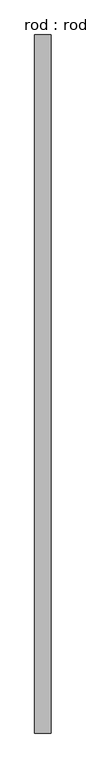
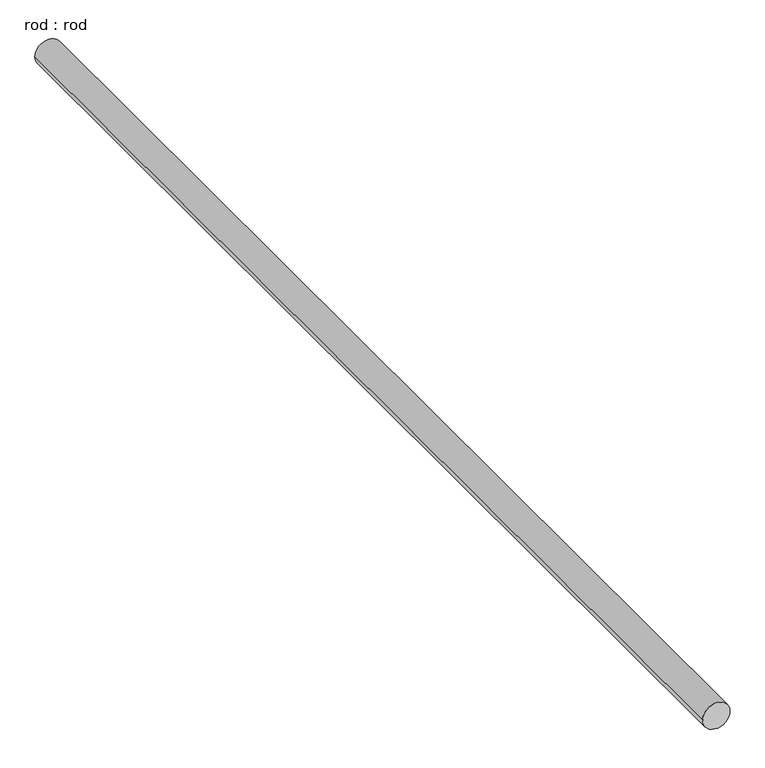
"""IFC4 building model written with IfcOpenShell, lengths in millimetres: proxy geometry, rod : rod."""

import ifcopenshell
import ifcopenshell.guid

model = None  # the IFC model being written
_history = None  # IfcOwnerHistory: only IFC2X3 demands one
_inside = {}  # id of a spatial element -> (the spatial element, [elements in it])
_under = {}  # id of a project, library or spatial element -> (it, [spatial elements below it])
_declared = {}  # id of a project -> (the project, [libraries it declares])
_typed = {}  # id of a type object -> (the type object, [elements of that type])
_made_of = {}  # id of a material, layer set ... -> (it, [elements and type objects made of it])


def new_model(schema):
    """Start an empty IFC model of exactly this schema.

    Asked for "IFC4X3", IfcOpenShell would pick the latest addendum, in which some entities
    have other attributes; the version numbers below select the first issue.
    IFC2X3 requires an IfcOwnerHistory on every rooted entity: one is made here for all.
    """
    global model, _history
    if schema == "IFC4X3":
        model = ifcopenshell.file(schema_version=(4, 3, 0, 0))
    else:
        model = ifcopenshell.file(schema=schema)
    _inside.clear()
    _under.clear()
    _declared.clear()
    _typed.clear()
    _made_of.clear()
    _history = None
    if model.schema == "IFC2X3":
        org = make("IfcOrganization", Name="unknown")
        user = make(
            "IfcPersonAndOrganization",
            ThePerson=make("IfcPerson", FamilyName="unknown"),
            TheOrganization=org,
        )
        app = make(
            "IfcApplication",
            ApplicationDeveloper=org,
            Version="unknown",
            ApplicationFullName="unknown",
            ApplicationIdentifier="unknown",
        )
        _history = make(
            "IfcOwnerHistory",
            OwningUser=user,
            OwningApplication=app,
            ChangeAction="ADDED",
            CreationDate=0,
        )
    return model


def make(cls, **values):
    """One entity of the class cls with the attributes given. An attribute that is None is left unset."""
    return model.create_entity(
        cls, **{name: value for name, value in values.items() if value is not None}
    )


def rooted(cls, **values):
    """An entity with a GlobalId (a new one), such as an element, a storey or a relation."""
    return make(cls, GlobalId=ifcopenshell.guid.new(), OwnerHistory=_history, **values)


def si_unit(unit_type, name, prefix=None):
    """IfcSIUnit, for example si_unit("LENGTHUNIT", "METRE", prefix="MILLI")."""
    return make("IfcSIUnit", UnitType=unit_type, Prefix=prefix, Name=name)


def assignment(units):
    """IfcUnitAssignment: the units of a project."""
    return None if units is None else make("IfcUnitAssignment", Units=units)


def point(xyz):
    """IfcCartesianPoint."""
    return None if xyz is None else make("IfcCartesianPoint", Coordinates=xyz)


def direction(xyz):
    """IfcDirection."""
    return None if xyz is None else make("IfcDirection", DirectionRatios=xyz)


def frame(location, z_axis=None, x_axis=None):
    """IfcAxis2Placement3D, a coordinate frame: its origin and axes. An axis left out is left unset."""
    return make(
        "IfcAxis2Placement3D",
        Location=point(location),
        Axis=direction(z_axis),
        RefDirection=direction(x_axis),
    )


def frame_2d(location, x_axis=None):
    """IfcAxis2Placement2D, a coordinate frame in the plane: its origin and x axis."""
    return make(
        "IfcAxis2Placement2D", Location=point(location), RefDirection=direction(x_axis)
    )


def origin():
    """The frame at (0, 0, 0) with its axes left unset."""
    return frame((0.0, 0.0, 0.0))


def place(relative_to, where):
    """IfcLocalPlacement: puts the frame where relative to a parent placement (None: the world)."""
    return make(
        "IfcLocalPlacement", PlacementRelTo=relative_to, RelativePlacement=where
    )


def context(
    kind, dimensions, precision=None, world=None, true_north=None, identifier=None
):
    """IfcGeometricRepresentationContext, for example the 3D "Model" context."""
    return make(
        "IfcGeometricRepresentationContext",
        ContextIdentifier=identifier,
        ContextType=kind,
        CoordinateSpaceDimension=dimensions,
        Precision=precision,
        WorldCoordinateSystem=world,
        TrueNorth=true_north,
    )


def project(units=None, contexts=None):
    """IfcProject with its units and contexts."""
    return rooted(
        "IfcProject",
        Name="project",
        RepresentationContexts=contexts,
        UnitsInContext=assignment(units),
    )


def spatial(cls, under=None, at=None, **own):
    """A site, building, storey or space (cls), placed at a placement, below another one or the project."""
    s = rooted(cls, ObjectPlacement=at, **own)
    if under is not None:
        _under.setdefault(under.id(), (under, []))[1].append(s)
    return s


def circle_curve(where, radius):
    """IfcCircle in the frame where."""
    return make("IfcCircle", Position=where, Radius=radius)


def trimmed(basis, trim1, trim2, sense, master):
    """IfcTrimmedCurve: the piece of a basis curve between two trims."""
    return make(
        "IfcTrimmedCurve",
        BasisCurve=basis,
        Trim1=trim1,
        Trim2=trim2,
        SenseAgreement=sense,
        MasterRepresentation=master,
    )


def segment(curve, same_sense, transition):
    """IfcCompositeCurveSegment."""
    return make(
        "IfcCompositeCurveSegment",
        Transition=transition,
        SameSense=same_sense,
        ParentCurve=curve,
    )


def composite_curve(segments, self_intersect=None):
    """IfcCompositeCurve: segments joined end to end."""
    return make("IfcCompositeCurve", Segments=segments, SelfIntersect=self_intersect)


def outline(outer, holes=None, kind="AREA"):
    """IfcArbitraryClosedProfileDef: a profile drawn as a closed curve; with holes, ...WithVoids."""
    if holes is None:
        return make("IfcArbitraryClosedProfileDef", ProfileType=kind, OuterCurve=outer)
    return make(
        "IfcArbitraryProfileDefWithVoids",
        ProfileType=kind,
        OuterCurve=outer,
        InnerCurves=holes,
    )


def extrude(swept, where, along, depth):
    """IfcExtrudedAreaSolid: the profile swept, set in the frame where, extruded along a direction by depth."""
    return make(
        "IfcExtrudedAreaSolid",
        SweptArea=swept,
        Position=where,
        ExtrudedDirection=direction(along),
        Depth=depth,
    )


def shape(context_of_items, identifier, shape_type, items):
    """IfcShapeRepresentation: the items that make up one representation, for example the "Body"."""
    return make(
        "IfcShapeRepresentation",
        ContextOfItems=context_of_items,
        RepresentationIdentifier=identifier,
        RepresentationType=shape_type,
        Items=items,
    )


def source(mapping_origin, context_of_items, identifier, shape_type, items):
    """IfcRepresentationMap: a shape defined once, which mapped items show again and again."""
    return make(
        "IfcRepresentationMap",
        MappingOrigin=mapping_origin,
        MappedRepresentation=shape(context_of_items, identifier, shape_type, items),
    )


def transform(
    local_origin,
    x_axis=None,
    y_axis=None,
    z_axis=None,
    scale=None,
    scale2=None,
    scale3=None,
    uniform=True,
):
    """IfcCartesianTransformationOperator3D, or its non-uniform kind. x_axis, y_axis, z_axis: its Axis1, 2, 3."""
    if uniform:
        return make(
            "IfcCartesianTransformationOperator3D",
            Axis1=direction(x_axis),
            Axis2=direction(y_axis),
            LocalOrigin=point(local_origin),
            Scale=scale,
            Axis3=direction(z_axis),
        )
    return make(
        "IfcCartesianTransformationOperator3DnonUniform",
        Axis1=direction(x_axis),
        Axis2=direction(y_axis),
        LocalOrigin=point(local_origin),
        Scale=scale,
        Axis3=direction(z_axis),
        Scale2=scale2,
        Scale3=scale3,
    )


def mapped(mapping_source, mapping_target):
    """IfcMappedItem: shows the shape of a source again, moved by a transform."""
    return make(
        "IfcMappedItem", MappingSource=mapping_source, MappingTarget=mapping_target
    )


def made_of(thing, what):
    """Note that an element or type object is made of a material, layer set ...; save() writes the relation."""
    if what is not None:
        _made_of.setdefault(what.id(), (what, []))[1].append(thing)
    return thing


def element(
    cls,
    number,
    at=None,
    inside=None,
    cuts=None,
    type_object=None,
    material=None,
    context=None,
    identifier="Body",
    shape_type=None,
    held_by="IfcProductDefinitionShape",
    body=None,
    shapes=None,
    **own,
):
    """One element of the class cls, such as IfcWall. Its Tag is "e" and its number.

    at: its placement. inside: the storey or other place that contains it. cuts: it is an
    opening in that element (IfcRelVoidsElement). A single representation is given by context,
    identifier, shape_type and body (its items); several are given by shapes. held_by: the class
    of the entity that holds the representations. save() writes the other relations.
    """
    e = rooted(cls, Tag="e%d" % number, ObjectPlacement=at, **own)
    if body is not None:
        shapes = [shape(context, identifier, shape_type, body)]
    if shapes is not None:
        e.Representation = make(held_by, Representations=shapes)
    if inside is not None:
        _inside.setdefault(inside.id(), (inside, []))[1].append(e)
    if cuts is not None:
        rooted(
            "IfcRelVoidsElement", RelatingBuildingElement=cuts, RelatedOpeningElement=e
        )
    if type_object is not None:
        _typed.setdefault(type_object.id(), (type_object, []))[1].append(e)
    return made_of(e, material)


def aggregate(whole, parts):
    """IfcRelAggregates: a whole, such as a stair, and the parts it consists of."""
    return rooted("IfcRelAggregates", RelatingObject=whole, RelatedObjects=parts)


def save(model, path):
    """Write the relations noted so far, then the file.

    IfcRelAggregates (storeys below a building ...), IfcRelContainedInSpatialStructure (elements
    in a storey), IfcRelDefinesByType, IfcRelAssociatesMaterial and IfcRelDeclares: one each for
    every whole, place, type object, material and project.
    """
    for whole, parts in _under.values():
        aggregate(whole, parts)
    for where, things in _inside.values():
        rooted(
            "IfcRelContainedInSpatialStructure",
            RelatedElements=things,
            RelatingStructure=where,
        )
    for kind, things in _typed.values():
        rooted("IfcRelDefinesByType", RelatedObjects=things, RelatingType=kind)
    for what, things in _made_of.values():
        rooted("IfcRelAssociatesMaterial", RelatedObjects=things, RelatingMaterial=what)
    for by, libraries in _declared.values():
        rooted("IfcRelDeclares", RelatingContext=by, RelatedDefinitions=libraries)
    model.write(path)


def rod_rod_a9224c9c(model_context):
    return source(origin(), model_context, "Body", "SweptSolid", [
        extrude(outline(composite_curve([segment(trimmed(circle_curve(frame_2d((0.0108462, 0.0)), 200.0), [point((0.0108462, 200.0))], [point((0.0108462, -200.0))], False, "CARTESIAN"), True, "CONTINUOUS"), segment(trimmed(circle_curve(frame_2d((0.0108462, 0.0)), 200.0), [point((0.0108462, -200.0))], [point((0.0108462, 200.0))], False, "CARTESIAN"), True, "CONTINUOUS")], self_intersect=False)), frame((0.0, -4398.5168763, 0.0), z_axis=(0.0, 1.0, 0.0), x_axis=(0.0, 0.0, 1.0)), (0.0, 0.0, 1.0), 16982.4909834),
    ])


if __name__ == "__main__":
    model = new_model("IFC4")
    model_context = context("Model", 3, world=origin())
    ifc_project = project(units=[si_unit("LENGTHUNIT", "METRE", prefix="MILLI")], contexts=[model_context])
    site = spatial("IfcSite", under=ifc_project)
    building = spatial("IfcBuilding", under=site)
    placement = place(None, origin())
    rod_rod_shape = rod_rod_a9224c9c(model_context)
    element("IfcBuildingElementProxy", 1, Name="rod : rod", ObjectType="rod : rod", at=placement, inside=building, context=model_context, shape_type="MappedRepresentation", body=[
        mapped(rod_rod_shape, transform((0.0, 0.0, 0.0), x_axis=(1.0, 0.0, 0.0), y_axis=(0.0, 1.0, 0.0), z_axis=(0.0, 0.0, 1.0))),
    ])
    save(model, "model.ifc")

# Revit data of these elements
# Type "rod : rod"
#   Default Elevation = 0
